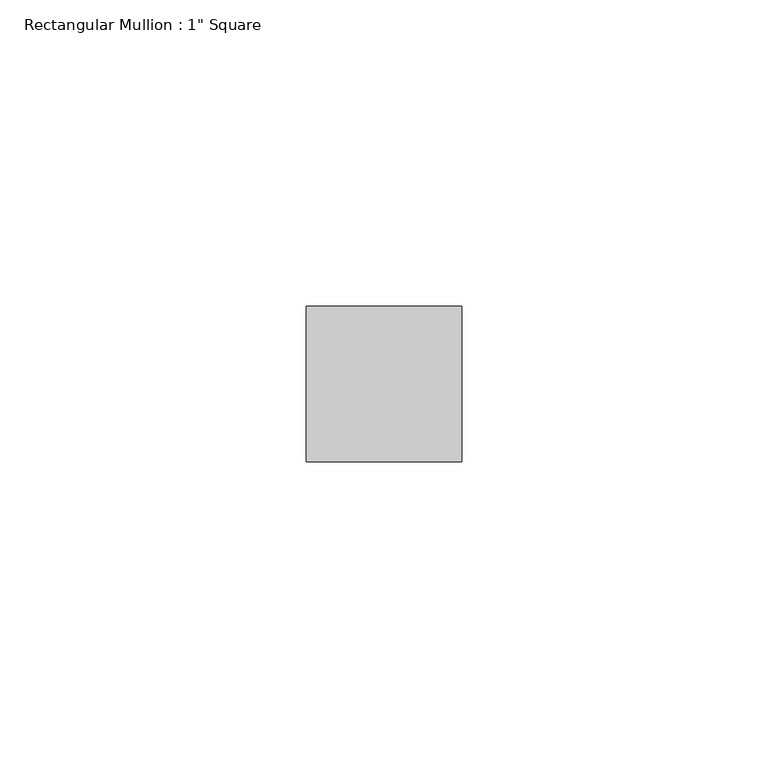
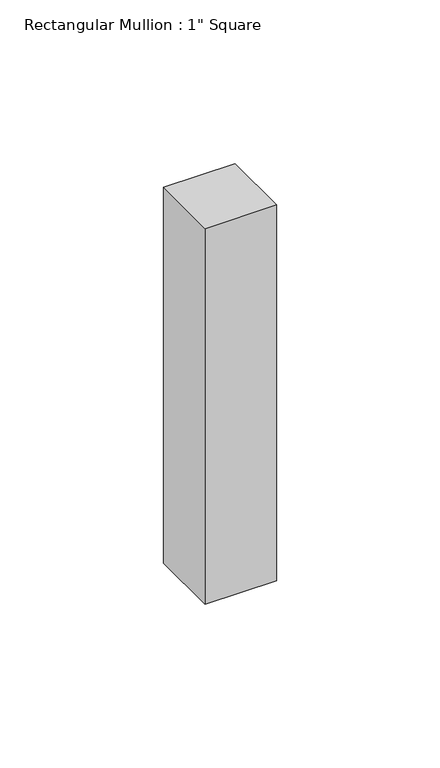
"""IFC4 building model written with IfcOpenShell, lengths in millimetres: member geometry."""

from ifc_helpers import new_model, si_unit, frame, origin, place, context, project, spatial, polyline, outline, extrude, source, transform, mapped, element, save


def member_89c5749c(model_context):
    return source(origin(), model_context, "Body", "SweptSolid", [
        extrude(outline(polyline([(0.0, 12.7), (0.0, -12.7), (-25.4, -12.7), (-25.4, 12.7), (0.0, 12.7)])), frame((0.0, 0.0, -140.3306552), z_axis=(0.0, 0.0, 1.0), x_axis=(1.0, 0.0, 0.0)), (0.0, 0.0, 1.0), 140.3306552),
    ])


if __name__ == "__main__":
    model = new_model("IFC4")
    model_context = context("Model", 3, world=origin())
    ifc_project = project(units=[si_unit("LENGTHUNIT", "METRE", prefix="MILLI")], contexts=[model_context])
    site = spatial("IfcSite", under=ifc_project)
    building = spatial("IfcBuilding", under=site)
    placement = place(None, origin())
    member_shape = member_89c5749c(model_context)
    element("IfcMember", 1, ObjectType="Rectangular Mullion : 1\" Square", at=placement, inside=building, context=model_context, shape_type="MappedRepresentation", body=[
        mapped(member_shape, transform((0.0, 0.0, 0.0), x_axis=(1.0, 0.0, 0.0), y_axis=(0.0, 1.0, 0.0), z_axis=(0.0, 0.0, 1.0))),
    ])
    save(model, "model.ifc")

# Revit data of these elements
# Type "Rectangular Mullion : 1\" Square"
#   built-in parameter 1007304 = 0.0833333 (stored number, unit not read)
#   built-in parameter 1007301 = 0.0416667 (stored number, unit not read)
#   built-in parameter 1007300 = 0.0416667 (stored number, unit not read)
# Element 1 (IfcMember, "Rectangular Mullion : 1\" Square")
#   Materials on its faces: "Metal - Aluminum"
# Materials
#   "Metal - Aluminum": class "Metal", colour RGB 247 247 247, transparency 0
